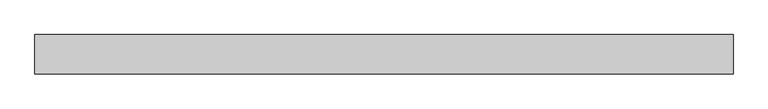
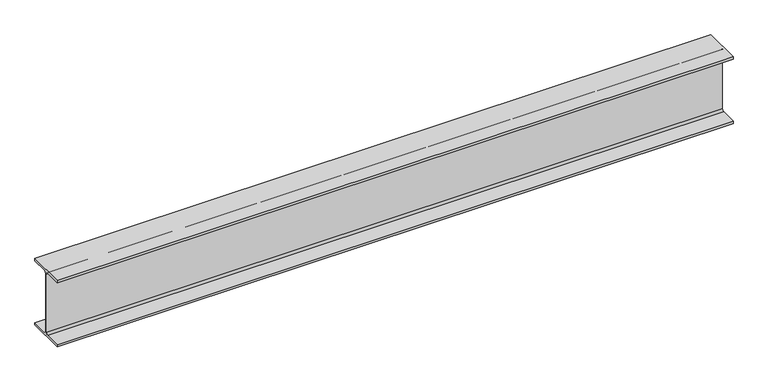
"""IFC4 building model written with IfcOpenShell, lengths in millimetres: beam geometry, Steel Beam_H-KSD3502 : H_SB_ASB_H-250x125x6x9."""

import ifcopenshell
import ifcopenshell.guid

model = None  # the IFC model being written
_history = None  # IfcOwnerHistory: only IFC2X3 demands one
_inside = {}  # id of a spatial element -> (the spatial element, [elements in it])
_under = {}  # id of a project, library or spatial element -> (it, [spatial elements below it])
_declared = {}  # id of a project -> (the project, [libraries it declares])
_typed = {}  # id of a type object -> (the type object, [elements of that type])
_made_of = {}  # id of a material, layer set ... -> (it, [elements and type objects made of it])


def new_model(schema):
    """Start an empty IFC model of exactly this schema.

    Asked for "IFC4X3", IfcOpenShell would pick the latest addendum, in which some entities
    have other attributes; the version numbers below select the first issue.
    IFC2X3 requires an IfcOwnerHistory on every rooted entity: one is made here for all.
    """
    global model, _history
    if schema == "IFC4X3":
        model = ifcopenshell.file(schema_version=(4, 3, 0, 0))
    else:
        model = ifcopenshell.file(schema=schema)
    _inside.clear()
    _under.clear()
    _declared.clear()
    _typed.clear()
    _made_of.clear()
    _history = None
    if model.schema == "IFC2X3":
        org = make("IfcOrganization", Name="unknown")
        user = make(
            "IfcPersonAndOrganization",
            ThePerson=make("IfcPerson", FamilyName="unknown"),
            TheOrganization=org,
        )
        app = make(
            "IfcApplication",
            ApplicationDeveloper=org,
            Version="unknown",
            ApplicationFullName="unknown",
            ApplicationIdentifier="unknown",
        )
        _history = make(
            "IfcOwnerHistory",
            OwningUser=user,
            OwningApplication=app,
            ChangeAction="ADDED",
            CreationDate=0,
        )
    return model


def make(cls, **values):
    """One entity of the class cls with the attributes given. An attribute that is None is left unset."""
    return model.create_entity(
        cls, **{name: value for name, value in values.items() if value is not None}
    )


def rooted(cls, **values):
    """An entity with a GlobalId (a new one), such as an element, a storey or a relation."""
    return make(cls, GlobalId=ifcopenshell.guid.new(), OwnerHistory=_history, **values)


def si_unit(unit_type, name, prefix=None):
    """IfcSIUnit, for example si_unit("LENGTHUNIT", "METRE", prefix="MILLI")."""
    return make("IfcSIUnit", UnitType=unit_type, Prefix=prefix, Name=name)


def assignment(units):
    """IfcUnitAssignment: the units of a project."""
    return None if units is None else make("IfcUnitAssignment", Units=units)


def point(xyz):
    """IfcCartesianPoint."""
    return None if xyz is None else make("IfcCartesianPoint", Coordinates=xyz)


def direction(xyz):
    """IfcDirection."""
    return None if xyz is None else make("IfcDirection", DirectionRatios=xyz)


def frame(location, z_axis=None, x_axis=None):
    """IfcAxis2Placement3D, a coordinate frame: its origin and axes. An axis left out is left unset."""
    return make(
        "IfcAxis2Placement3D",
        Location=point(location),
        Axis=direction(z_axis),
        RefDirection=direction(x_axis),
    )


def frame_2d(location, x_axis=None):
    """IfcAxis2Placement2D, a coordinate frame in the plane: its origin and x axis."""
    return make(
        "IfcAxis2Placement2D", Location=point(location), RefDirection=direction(x_axis)
    )


def origin():
    """The frame at (0, 0, 0) with its axes left unset."""
    return frame((0.0, 0.0, 0.0))


def place(relative_to, where):
    """IfcLocalPlacement: puts the frame where relative to a parent placement (None: the world)."""
    return make(
        "IfcLocalPlacement", PlacementRelTo=relative_to, RelativePlacement=where
    )


def context(
    kind, dimensions, precision=None, world=None, true_north=None, identifier=None
):
    """IfcGeometricRepresentationContext, for example the 3D "Model" context."""
    return make(
        "IfcGeometricRepresentationContext",
        ContextIdentifier=identifier,
        ContextType=kind,
        CoordinateSpaceDimension=dimensions,
        Precision=precision,
        WorldCoordinateSystem=world,
        TrueNorth=true_north,
    )


def project(units=None, contexts=None):
    """IfcProject with its units and contexts."""
    return rooted(
        "IfcProject",
        Name="project",
        RepresentationContexts=contexts,
        UnitsInContext=assignment(units),
    )


def spatial(cls, under=None, at=None, **own):
    """A site, building, storey or space (cls), placed at a placement, below another one or the project."""
    s = rooted(cls, ObjectPlacement=at, **own)
    if under is not None:
        _under.setdefault(under.id(), (under, []))[1].append(s)
    return s


def polyline(points):
    """IfcPolyline through the points."""
    return make("IfcPolyline", Points=[point(p) for p in points])


def circle_curve(where, radius):
    """IfcCircle in the frame where."""
    return make("IfcCircle", Position=where, Radius=radius)


def trimmed(basis, trim1, trim2, sense, master):
    """IfcTrimmedCurve: the piece of a basis curve between two trims."""
    return make(
        "IfcTrimmedCurve",
        BasisCurve=basis,
        Trim1=trim1,
        Trim2=trim2,
        SenseAgreement=sense,
        MasterRepresentation=master,
    )


def segment(curve, same_sense, transition):
    """IfcCompositeCurveSegment."""
    return make(
        "IfcCompositeCurveSegment",
        Transition=transition,
        SameSense=same_sense,
        ParentCurve=curve,
    )


def composite_curve(segments, self_intersect=None):
    """IfcCompositeCurve: segments joined end to end."""
    return make("IfcCompositeCurve", Segments=segments, SelfIntersect=self_intersect)


def outline(outer, holes=None, kind="AREA"):
    """IfcArbitraryClosedProfileDef: a profile drawn as a closed curve; with holes, ...WithVoids."""
    if holes is None:
        return make("IfcArbitraryClosedProfileDef", ProfileType=kind, OuterCurve=outer)
    return make(
        "IfcArbitraryProfileDefWithVoids",
        ProfileType=kind,
        OuterCurve=outer,
        InnerCurves=holes,
    )


def extrude(swept, where, along, depth):
    """IfcExtrudedAreaSolid: the profile swept, set in the frame where, extruded along a direction by depth."""
    return make(
        "IfcExtrudedAreaSolid",
        SweptArea=swept,
        Position=where,
        ExtrudedDirection=direction(along),
        Depth=depth,
    )


def shape(context_of_items, identifier, shape_type, items):
    """IfcShapeRepresentation: the items that make up one representation, for example the "Body"."""
    return make(
        "IfcShapeRepresentation",
        ContextOfItems=context_of_items,
        RepresentationIdentifier=identifier,
        RepresentationType=shape_type,
        Items=items,
    )


def source(mapping_origin, context_of_items, identifier, shape_type, items):
    """IfcRepresentationMap: a shape defined once, which mapped items show again and again."""
    return make(
        "IfcRepresentationMap",
        MappingOrigin=mapping_origin,
        MappedRepresentation=shape(context_of_items, identifier, shape_type, items),
    )


def transform(
    local_origin,
    x_axis=None,
    y_axis=None,
    z_axis=None,
    scale=None,
    scale2=None,
    scale3=None,
    uniform=True,
):
    """IfcCartesianTransformationOperator3D, or its non-uniform kind. x_axis, y_axis, z_axis: its Axis1, 2, 3."""
    if uniform:
        return make(
            "IfcCartesianTransformationOperator3D",
            Axis1=direction(x_axis),
            Axis2=direction(y_axis),
            LocalOrigin=point(local_origin),
            Scale=scale,
            Axis3=direction(z_axis),
        )
    return make(
        "IfcCartesianTransformationOperator3DnonUniform",
        Axis1=direction(x_axis),
        Axis2=direction(y_axis),
        LocalOrigin=point(local_origin),
        Scale=scale,
        Axis3=direction(z_axis),
        Scale2=scale2,
        Scale3=scale3,
    )


def mapped(mapping_source, mapping_target):
    """IfcMappedItem: shows the shape of a source again, moved by a transform."""
    return make(
        "IfcMappedItem", MappingSource=mapping_source, MappingTarget=mapping_target
    )


def made_of(thing, what):
    """Note that an element or type object is made of a material, layer set ...; save() writes the relation."""
    if what is not None:
        _made_of.setdefault(what.id(), (what, []))[1].append(thing)
    return thing


def element(
    cls,
    number,
    at=None,
    inside=None,
    cuts=None,
    type_object=None,
    material=None,
    context=None,
    identifier="Body",
    shape_type=None,
    held_by="IfcProductDefinitionShape",
    body=None,
    shapes=None,
    **own,
):
    """One element of the class cls, such as IfcWall. Its Tag is "e" and its number.

    at: its placement. inside: the storey or other place that contains it. cuts: it is an
    opening in that element (IfcRelVoidsElement). A single representation is given by context,
    identifier, shape_type and body (its items); several are given by shapes. held_by: the class
    of the entity that holds the representations. save() writes the other relations.
    """
    e = rooted(cls, Tag="e%d" % number, ObjectPlacement=at, **own)
    if body is not None:
        shapes = [shape(context, identifier, shape_type, body)]
    if shapes is not None:
        e.Representation = make(held_by, Representations=shapes)
    if inside is not None:
        _inside.setdefault(inside.id(), (inside, []))[1].append(e)
    if cuts is not None:
        rooted(
            "IfcRelVoidsElement", RelatingBuildingElement=cuts, RelatedOpeningElement=e
        )
    if type_object is not None:
        _typed.setdefault(type_object.id(), (type_object, []))[1].append(e)
    return made_of(e, material)


def aggregate(whole, parts):
    """IfcRelAggregates: a whole, such as a stair, and the parts it consists of."""
    return rooted("IfcRelAggregates", RelatingObject=whole, RelatedObjects=parts)


def save(model, path):
    """Write the relations noted so far, then the file.

    IfcRelAggregates (storeys below a building ...), IfcRelContainedInSpatialStructure (elements
    in a storey), IfcRelDefinesByType, IfcRelAssociatesMaterial and IfcRelDeclares: one each for
    every whole, place, type object, material and project.
    """
    for whole, parts in _under.values():
        aggregate(whole, parts)
    for where, things in _inside.values():
        rooted(
            "IfcRelContainedInSpatialStructure",
            RelatedElements=things,
            RelatingStructure=where,
        )
    for kind, things in _typed.values():
        rooted("IfcRelDefinesByType", RelatedObjects=things, RelatingType=kind)
    for what, things in _made_of.values():
        rooted("IfcRelAssociatesMaterial", RelatedObjects=things, RelatingMaterial=what)
    for by, libraries in _declared.values():
        rooted("IfcRelDeclares", RelatingContext=by, RelatedDefinitions=libraries)
    model.write(path)


def beam_201670e7(model_context):
    return source(origin(), model_context, "Body", "SweptSolid", [
        extrude(outline(composite_curve([segment(polyline([(82.5, -141.5), (82.5, -151.7), (-82.5, -151.7), (-82.5, -141.5), (-11.9, -141.5)]), True, "CONTINUOUS"), segment(trimmed(circle_curve(frame_2d((-11.9, -132.6)), 8.9), [point((-11.9, -141.5))], [point((-3.0, -132.6))], True, "CARTESIAN"), True, "CONTINUOUS"), segment(polyline([(-3.0, -132.6), (-3.0, 132.6)]), True, "CONTINUOUS"), segment(trimmed(circle_curve(frame_2d((-11.9, 132.6)), 8.9), [point((-3.0, 132.6))], [point((-11.9, 141.5))], True, "CARTESIAN"), True, "CONTINUOUS"), segment(polyline([(-11.9, 141.5), (-82.5, 141.5), (-82.5, 151.7), (82.5, 151.7), (82.5, 141.5), (11.9, 141.5)]), True, "CONTINUOUS"), segment(trimmed(circle_curve(frame_2d((11.9, 132.6)), 8.9), [point((11.9, 141.5))], [point((3.0, 132.6))], True, "CARTESIAN"), True, "CONTINUOUS"), segment(polyline([(3.0, 132.6), (3.0, -132.6)]), True, "CONTINUOUS"), segment(trimmed(circle_curve(frame_2d((11.9, -132.6)), 8.9), [point((3.0, -132.6))], [point((11.9, -141.5))], True, "CARTESIAN"), True, "CONTINUOUS"), segment(polyline([(11.9, -141.5), (82.5, -141.5)]), True, "CONTINUOUS")], self_intersect=False)), frame((-1529.8, 0.0, 0.0), z_axis=(1.0, 0.0, 0.0), x_axis=(0.0, 1.0, 0.0)), (0.0, 0.0, 1.0), 2912.1488581),
    ])


if __name__ == "__main__":
    model = new_model("IFC4")
    model_context = context("Model", 3, world=origin())
    ifc_project = project(units=[si_unit("LENGTHUNIT", "METRE", prefix="MILLI")], contexts=[model_context])
    site = spatial("IfcSite", under=ifc_project)
    building = spatial("IfcBuilding", under=site)
    placement = place(None, origin())
    beam_shape = beam_201670e7(model_context)
    element("IfcBeam", 1, ObjectType="Steel Beam_H-KSD3502 : H_SB_ASB_H-250x125x6x9", at=placement, inside=building, context=model_context, shape_type="MappedRepresentation", body=[
        mapped(beam_shape, transform((0.0, 0.0, 0.0), x_axis=(1.0, 0.0, 0.0), y_axis=(0.0, 1.0, 0.0), z_axis=(0.0, 0.0, 1.0))),
    ])
    save(model, "model.ifc")

# Revit data of these elements
# Type "Steel Beam_H-KSD3502 : H_SB_ASB_H-250x125x6x9"
#   Width = 12.5 cm
#   Web Thickness = 0.6 cm
#   Web Fillet = 1.2 cm
#   Warping Constant = 42539.8 cm⁶
#   Torsional Moment of Inertia = 7.8102 cm⁴
#   Torsional Modulus = 1.0 cm³
#   Section Area = 37.66 cm²
#   Plastic Modulus weak axis = 73.1 cm³
#   Plastic Modulus strong axis = 366.0 cm³
#   Perimeter = 0.97 m²/m
#   Nominal Weight = 29.60 kgf/m
#   Moment of Inertia weak axis = 294.00 cm⁴
#   Moment of Inertia strong axis = 4050.00 cm⁴
#   Height = 25.0 cm
#   Flange Thickness = 0.9 cm
#   Elastic Modulus weak axis = 47.0 cm³
#   Elastic Modulus strong axis = 324.0 cm³
#   Centroid Vertical = 12.5 cm
#   Centroid Horizontal = 6.25 cm
#   Length [instance default] = 1.5240 m
#   Structural Material [instance default] = Steel, 45-345
#   Assembly Code = ""
# Element 1 (IfcBeam, "Steel Beam_H-KSD3502 : H_SB_ASB_H-250x125x6x9")
#   Structural Material = none
# Materials
#   "Steel, 45-345": class "Metal", colour RGB 189 187 185, transparency 0, Description = "Steel 345 MPa", Cost = 0
